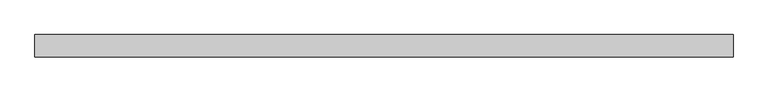
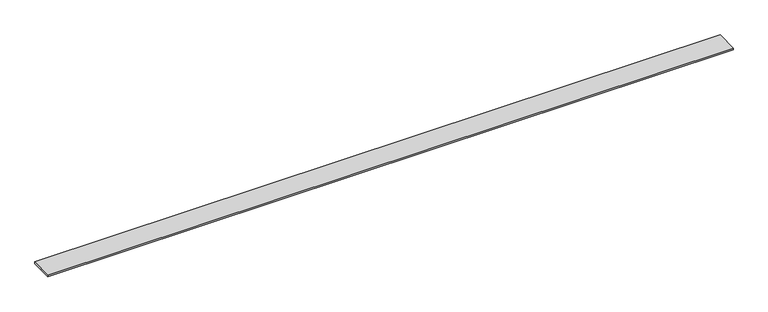
"""IFC4 building model written with IfcOpenShell, lengths in millimetres: proxy geometry, Generic Models 7:Generic Models 1:2:Generic Models 1:2 : Generic Models 7:Generic Models 1:337419:8 : Generic Models 7:Generic Models 1:2:Generic Models 1:2 : Generic Models 7:Generic Models 1:337419:306751."""

import ifcopenshell
import ifcopenshell.guid

model = None  # the IFC model being written
_history = None  # IfcOwnerHistory: only IFC2X3 demands one
_inside = {}  # id of a spatial element -> (the spatial element, [elements in it])
_under = {}  # id of a project, library or spatial element -> (it, [spatial elements below it])
_declared = {}  # id of a project -> (the project, [libraries it declares])
_typed = {}  # id of a type object -> (the type object, [elements of that type])
_made_of = {}  # id of a material, layer set ... -> (it, [elements and type objects made of it])


def new_model(schema):
    """Start an empty IFC model of exactly this schema.

    Asked for "IFC4X3", IfcOpenShell would pick the latest addendum, in which some entities
    have other attributes; the version numbers below select the first issue.
    IFC2X3 requires an IfcOwnerHistory on every rooted entity: one is made here for all.
    """
    global model, _history
    if schema == "IFC4X3":
        model = ifcopenshell.file(schema_version=(4, 3, 0, 0))
    else:
        model = ifcopenshell.file(schema=schema)
    _inside.clear()
    _under.clear()
    _declared.clear()
    _typed.clear()
    _made_of.clear()
    _history = None
    if model.schema == "IFC2X3":
        org = make("IfcOrganization", Name="unknown")
        user = make(
            "IfcPersonAndOrganization",
            ThePerson=make("IfcPerson", FamilyName="unknown"),
            TheOrganization=org,
        )
        app = make(
            "IfcApplication",
            ApplicationDeveloper=org,
            Version="unknown",
            ApplicationFullName="unknown",
            ApplicationIdentifier="unknown",
        )
        _history = make(
            "IfcOwnerHistory",
            OwningUser=user,
            OwningApplication=app,
            ChangeAction="ADDED",
            CreationDate=0,
        )
    return model


def make(cls, **values):
    """One entity of the class cls with the attributes given. An attribute that is None is left unset."""
    return model.create_entity(
        cls, **{name: value for name, value in values.items() if value is not None}
    )


def rooted(cls, **values):
    """An entity with a GlobalId (a new one), such as an element, a storey or a relation."""
    return make(cls, GlobalId=ifcopenshell.guid.new(), OwnerHistory=_history, **values)


def si_unit(unit_type, name, prefix=None):
    """IfcSIUnit, for example si_unit("LENGTHUNIT", "METRE", prefix="MILLI")."""
    return make("IfcSIUnit", UnitType=unit_type, Prefix=prefix, Name=name)


def assignment(units):
    """IfcUnitAssignment: the units of a project."""
    return None if units is None else make("IfcUnitAssignment", Units=units)


def point(xyz):
    """IfcCartesianPoint."""
    return None if xyz is None else make("IfcCartesianPoint", Coordinates=xyz)


def direction(xyz):
    """IfcDirection."""
    return None if xyz is None else make("IfcDirection", DirectionRatios=xyz)


def frame(location, z_axis=None, x_axis=None):
    """IfcAxis2Placement3D, a coordinate frame: its origin and axes. An axis left out is left unset."""
    return make(
        "IfcAxis2Placement3D",
        Location=point(location),
        Axis=direction(z_axis),
        RefDirection=direction(x_axis),
    )


def origin():
    """The frame at (0, 0, 0) with its axes left unset."""
    return frame((0.0, 0.0, 0.0))


def place(relative_to, where):
    """IfcLocalPlacement: puts the frame where relative to a parent placement (None: the world)."""
    return make(
        "IfcLocalPlacement", PlacementRelTo=relative_to, RelativePlacement=where
    )


def context(
    kind, dimensions, precision=None, world=None, true_north=None, identifier=None
):
    """IfcGeometricRepresentationContext, for example the 3D "Model" context."""
    return make(
        "IfcGeometricRepresentationContext",
        ContextIdentifier=identifier,
        ContextType=kind,
        CoordinateSpaceDimension=dimensions,
        Precision=precision,
        WorldCoordinateSystem=world,
        TrueNorth=true_north,
    )


def project(units=None, contexts=None):
    """IfcProject with its units and contexts."""
    return rooted(
        "IfcProject",
        Name="project",
        RepresentationContexts=contexts,
        UnitsInContext=assignment(units),
    )


def spatial(cls, under=None, at=None, **own):
    """A site, building, storey or space (cls), placed at a placement, below another one or the project."""
    s = rooted(cls, ObjectPlacement=at, **own)
    if under is not None:
        _under.setdefault(under.id(), (under, []))[1].append(s)
    return s


def polyline(points):
    """IfcPolyline through the points."""
    return make("IfcPolyline", Points=[point(p) for p in points])


def outline(outer, holes=None, kind="AREA"):
    """IfcArbitraryClosedProfileDef: a profile drawn as a closed curve; with holes, ...WithVoids."""
    if holes is None:
        return make("IfcArbitraryClosedProfileDef", ProfileType=kind, OuterCurve=outer)
    return make(
        "IfcArbitraryProfileDefWithVoids",
        ProfileType=kind,
        OuterCurve=outer,
        InnerCurves=holes,
    )


def extrude(swept, where, along, depth):
    """IfcExtrudedAreaSolid: the profile swept, set in the frame where, extruded along a direction by depth."""
    return make(
        "IfcExtrudedAreaSolid",
        SweptArea=swept,
        Position=where,
        ExtrudedDirection=direction(along),
        Depth=depth,
    )


def shape(context_of_items, identifier, shape_type, items):
    """IfcShapeRepresentation: the items that make up one representation, for example the "Body"."""
    return make(
        "IfcShapeRepresentation",
        ContextOfItems=context_of_items,
        RepresentationIdentifier=identifier,
        RepresentationType=shape_type,
        Items=items,
    )


def source(mapping_origin, context_of_items, identifier, shape_type, items):
    """IfcRepresentationMap: a shape defined once, which mapped items show again and again."""
    return make(
        "IfcRepresentationMap",
        MappingOrigin=mapping_origin,
        MappedRepresentation=shape(context_of_items, identifier, shape_type, items),
    )


def transform(
    local_origin,
    x_axis=None,
    y_axis=None,
    z_axis=None,
    scale=None,
    scale2=None,
    scale3=None,
    uniform=True,
):
    """IfcCartesianTransformationOperator3D, or its non-uniform kind. x_axis, y_axis, z_axis: its Axis1, 2, 3."""
    if uniform:
        return make(
            "IfcCartesianTransformationOperator3D",
            Axis1=direction(x_axis),
            Axis2=direction(y_axis),
            LocalOrigin=point(local_origin),
            Scale=scale,
            Axis3=direction(z_axis),
        )
    return make(
        "IfcCartesianTransformationOperator3DnonUniform",
        Axis1=direction(x_axis),
        Axis2=direction(y_axis),
        LocalOrigin=point(local_origin),
        Scale=scale,
        Axis3=direction(z_axis),
        Scale2=scale2,
        Scale3=scale3,
    )


def mapped(mapping_source, mapping_target):
    """IfcMappedItem: shows the shape of a source again, moved by a transform."""
    return make(
        "IfcMappedItem", MappingSource=mapping_source, MappingTarget=mapping_target
    )


def made_of(thing, what):
    """Note that an element or type object is made of a material, layer set ...; save() writes the relation."""
    if what is not None:
        _made_of.setdefault(what.id(), (what, []))[1].append(thing)
    return thing


def element(
    cls,
    number,
    at=None,
    inside=None,
    cuts=None,
    type_object=None,
    material=None,
    context=None,
    identifier="Body",
    shape_type=None,
    held_by="IfcProductDefinitionShape",
    body=None,
    shapes=None,
    **own,
):
    """One element of the class cls, such as IfcWall. Its Tag is "e" and its number.

    at: its placement. inside: the storey or other place that contains it. cuts: it is an
    opening in that element (IfcRelVoidsElement). A single representation is given by context,
    identifier, shape_type and body (its items); several are given by shapes. held_by: the class
    of the entity that holds the representations. save() writes the other relations.
    """
    e = rooted(cls, Tag="e%d" % number, ObjectPlacement=at, **own)
    if body is not None:
        shapes = [shape(context, identifier, shape_type, body)]
    if shapes is not None:
        e.Representation = make(held_by, Representations=shapes)
    if inside is not None:
        _inside.setdefault(inside.id(), (inside, []))[1].append(e)
    if cuts is not None:
        rooted(
            "IfcRelVoidsElement", RelatingBuildingElement=cuts, RelatedOpeningElement=e
        )
    if type_object is not None:
        _typed.setdefault(type_object.id(), (type_object, []))[1].append(e)
    return made_of(e, material)


def aggregate(whole, parts):
    """IfcRelAggregates: a whole, such as a stair, and the parts it consists of."""
    return rooted("IfcRelAggregates", RelatingObject=whole, RelatedObjects=parts)


def save(model, path):
    """Write the relations noted so far, then the file.

    IfcRelAggregates (storeys below a building ...), IfcRelContainedInSpatialStructure (elements
    in a storey), IfcRelDefinesByType, IfcRelAssociatesMaterial and IfcRelDeclares: one each for
    every whole, place, type object, material and project.
    """
    for whole, parts in _under.values():
        aggregate(whole, parts)
    for where, things in _inside.values():
        rooted(
            "IfcRelContainedInSpatialStructure",
            RelatedElements=things,
            RelatingStructure=where,
        )
    for kind, things in _typed.values():
        rooted("IfcRelDefinesByType", RelatedObjects=things, RelatingType=kind)
    for what, things in _made_of.values():
        rooted("IfcRelAssociatesMaterial", RelatedObjects=things, RelatingMaterial=what)
    for by, libraries in _declared.values():
        rooted("IfcRelDeclares", RelatingContext=by, RelatedDefinitions=libraries)
    model.write(path)


def generic_models_a389b6f9(model_context):
    return source(origin(), model_context, "Body", "SweptSolid", [
        extrude(outline(polyline([(-578769.3946002, 3718.3565048), (-578769.8833674, 3730.7170007), (-578614.4535455, 3737.1932433), (-578613.9517445, 3724.5031321), (-578769.3946002, 3718.3565048)])), frame((591306.0367239, 0.0, 0.0), z_axis=(1.0, 0.0, 0.0), x_axis=(0.0, 1.0, 0.0)), (0.0, 0.0, 1.0), 4876.8),
    ])


if __name__ == "__main__":
    model = new_model("IFC4")
    model_context = context("Model", 3, world=origin())
    ifc_project = project(units=[si_unit("LENGTHUNIT", "METRE", prefix="MILLI")], contexts=[model_context])
    site = spatial("IfcSite", under=ifc_project)
    building = spatial("IfcBuilding", under=site)
    placement = place(None, origin())
    generic_models_shape = generic_models_a389b6f9(model_context)
    element("IfcBuildingElementProxy", 1, Name="Generic Models 7:Generic Models 1:2:Generic Models 1:2 : Generic Models 7:Generic Models 1:337419:8 : Generic Models 7:Generic Models 1:2:Generic Models 1:2 : Generic Models 7:Generic Models 1:337419:306751", ObjectType="Generic Models 7:Generic Models 1:2:Generic Models 1:2 : Generic Models 7:Generic Models 1:337419:8 : Generic Models 7:Generic Models 1:2:Generic Models 1:2 : Generic Models 7:Generic Models 1:337419:306751", at=placement, inside=building, context=model_context, shape_type="MappedRepresentation", body=[
        mapped(generic_models_shape, transform((0.0, 0.0, 0.0), x_axis=(1.0, 0.0, 0.0), y_axis=(0.0, 1.0, 0.0), z_axis=(0.0, 0.0, 1.0))),
    ])
    save(model, "model.ifc")

# Revit data of these elements
# Type "Generic Models 7:Generic Models 1:2:Generic Models 1:2 : Generic Models 7:Generic Models 1:337419:8 : Generic Models 7:Generic Models 1:2:Generic Models 1:2 : Generic Models 7:Generic Models 1:337419:306751"
#   NameOverride = "Generic Models 7:Generic Models 1:2:Generic Models 1:2 : Generic Models 7:Generic Models 1:337419:306751"
#   ObjectTypeOverride = "Generic Models 1:2 : Generic Models 7:Generic Models 1:337419"
#   Reference = "Generic Models 1"
#   Tag = "306751"
# Element 1 (IfcBuildingElementProxy, "Generic Models 7:Generic Models 1:2:Generic Models 1:2 : Generic Models 7:Generic Models 1:337419:8 : Generic Models 7:Generic Models 1:2:Generic Models 1:2 : Generic Models 7:Generic Models 1:337419:306751")
#   Materials on its faces: "FIRE RETARDTANT WOOD BLOCKING - SIZE AS NEC."
# Materials
#   "FIRE RETARDTANT WOOD BLOCKING - SIZE AS NEC.": class "Wood", colour RGB 144 113 62, transparency 0, Description = "Pinus Echinata", Cost = 0
